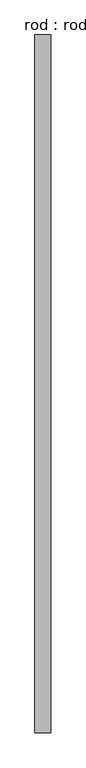
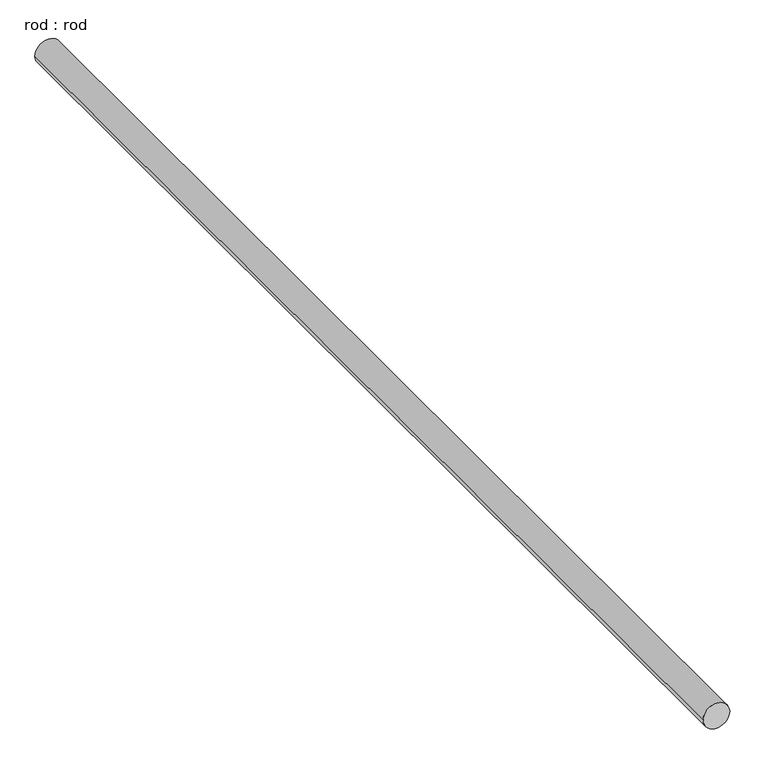
"""IFC4 building model written with IfcOpenShell, lengths in millimetres: proxy geometry, rod : rod."""

from ifc_helpers import new_model, si_unit, point, frame, frame_2d, origin, place, context, project, spatial, circle_curve, trimmed, segment, composite_curve, outline, extrude, source, transform, mapped, element, save


def rod_rod_15d19f25(model_context):
    return source(origin(), model_context, "Body", "SweptSolid", [
        extrude(outline(composite_curve([segment(trimmed(circle_curve(frame_2d((0.0108462, 0.0)), 200.0), [point((0.0108462, 200.0))], [point((0.0108462, -200.0))], False, "CARTESIAN"), True, "CONTINUOUS"), segment(trimmed(circle_curve(frame_2d((0.0108462, 0.0)), 200.0), [point((0.0108462, -200.0))], [point((0.0108462, 200.0))], False, "CARTESIAN"), True, "CONTINUOUS")], self_intersect=False)), frame((0.0, -4643.8786352, 0.0), z_axis=(0.0, 1.0, 0.0), x_axis=(0.0, 0.0, 1.0)), (0.0, 0.0, 1.0), 17473.2145011),
    ])


if __name__ == "__main__":
    model = new_model("IFC4")
    model_context = context("Model", 3, world=origin())
    ifc_project = project(units=[si_unit("LENGTHUNIT", "METRE", prefix="MILLI")], contexts=[model_context])
    site = spatial("IfcSite", under=ifc_project)
    building = spatial("IfcBuilding", under=site)
    placement = place(None, origin())
    rod_rod_shape = rod_rod_15d19f25(model_context)
    element("IfcBuildingElementProxy", 1, Name="rod : rod", ObjectType="rod : rod", at=placement, inside=building, context=model_context, shape_type="MappedRepresentation", body=[
        mapped(rod_rod_shape, transform((0.0, 0.0, 0.0), x_axis=(1.0, 0.0, 0.0), y_axis=(0.0, 1.0, 0.0), z_axis=(0.0, 0.0, 1.0))),
    ])
    save(model, "model.ifc")

# Revit data of these elements
# Type "rod : rod"
#   Default Elevation = 0
